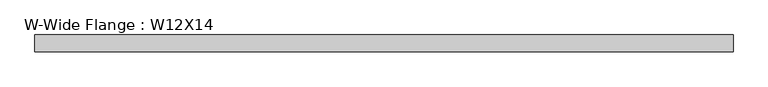
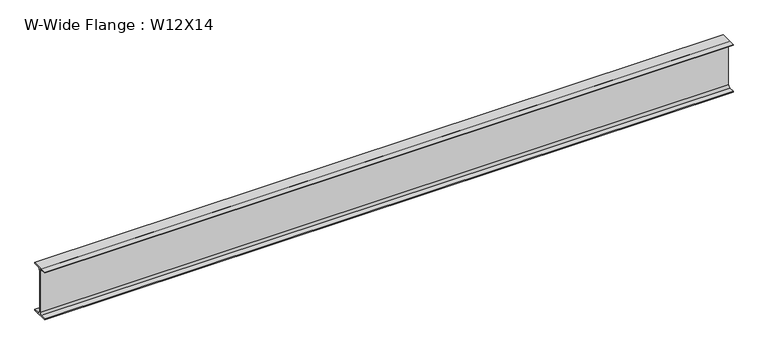
"""IFC4 building model written with IfcOpenShell, lengths in millimetres: beam geometry, W-Wide Flange : W12X14."""

from ifc_helpers import new_model, si_unit, point, frame, frame_2d, origin, place, context, project, spatial, polyline, circle_curve, trimmed, segment, composite_curve, outline, extrude, source, transform, mapped, element, save


def w_wide_flange_w12x14_653fb77d(model_context):
    return source(origin(), model_context, "Body", "SweptSolid", [
        extrude(outline(composite_curve([segment(polyline([(50.419, -145.415), (50.419, -151.13), (-50.419, -151.13), (-50.419, -145.415), (-15.875, -145.415)]), True, "CONTINUOUS"), segment(trimmed(circle_curve(frame_2d((-15.875, -132.08)), 13.335), [point((-15.875, -145.415))], [point((-2.54, -132.08))], True, "CARTESIAN"), True, "CONTINUOUS"), segment(polyline([(-2.54, -132.08), (-2.54, 132.08)]), True, "CONTINUOUS"), segment(trimmed(circle_curve(frame_2d((-15.875, 132.08)), 13.335), [point((-2.54, 132.08))], [point((-15.875, 145.415))], True, "CARTESIAN"), True, "CONTINUOUS"), segment(polyline([(-15.875, 145.415), (-50.419, 145.415), (-50.419, 151.13), (50.419, 151.13), (50.419, 145.415), (15.875, 145.415)]), True, "CONTINUOUS"), segment(trimmed(circle_curve(frame_2d((15.875, 132.08)), 13.335), [point((15.875, 145.415))], [point((2.54, 132.08))], True, "CARTESIAN"), True, "CONTINUOUS"), segment(polyline([(2.54, 132.08), (2.54, -132.08)]), True, "CONTINUOUS"), segment(trimmed(circle_curve(frame_2d((15.875, -132.08)), 13.335), [point((2.54, -132.08))], [point((15.875, -145.415))], True, "CARTESIAN"), True, "CONTINUOUS"), segment(polyline([(15.875, -145.415), (50.419, -145.415)]), True, "CONTINUOUS")], self_intersect=False)), frame((-2090.4727608, 0.0, 0.0), z_axis=(1.0, 0.0, 0.0), x_axis=(0.0, 1.0, 0.0)), (0.0, 0.0, 1.0), 4130.1824413),
    ])


if __name__ == "__main__":
    model = new_model("IFC4")
    model_context = context("Model", 3, world=origin())
    ifc_project = project(units=[si_unit("LENGTHUNIT", "METRE", prefix="MILLI")], contexts=[model_context])
    site = spatial("IfcSite", under=ifc_project)
    building = spatial("IfcBuilding", under=site)
    placement = place(None, origin())
    w_wide_flange_w12x14_shape = w_wide_flange_w12x14_653fb77d(model_context)
    element("IfcBeam", 1, ObjectType="W-Wide Flange : W12X14", at=placement, inside=building, context=model_context, shape_type="MappedRepresentation", body=[
        mapped(w_wide_flange_w12x14_shape, transform((0.0, 0.0, 0.0), x_axis=(1.0, 0.0, 0.0), y_axis=(0.0, 1.0, 0.0), z_axis=(0.0, 0.0, 1.0))),
    ])
    save(model, "model.ifc")

# Revit data of these elements
# Type "W-Wide Flange : W12X14"
#   Assembly Code = "B10"
#   W = 14
#   Length [instance default] = 5' - 0"
#   bf = 0' - 3.97"
#   d = 0' - 11.9"
#   k = 0' - 0 3/4"
#   k2 = 0' - 0.525"
#   tf = 0' - 0.225"
#   tw = 0' - 0.2"
#   A = 0.0288889 SF
#   Structural Material [instance default] = Steel ASTM A992
# Element 1 (IfcBeam, "W-Wide Flange : W12X14")
#   Materials on its faces: "Steel ASTM A992"
# Materials
#   "Steel ASTM A992": class "Metal", colour RGB 199 199 199, transparency 0, Description = "Structural steel 50ksi", Cost = 0
